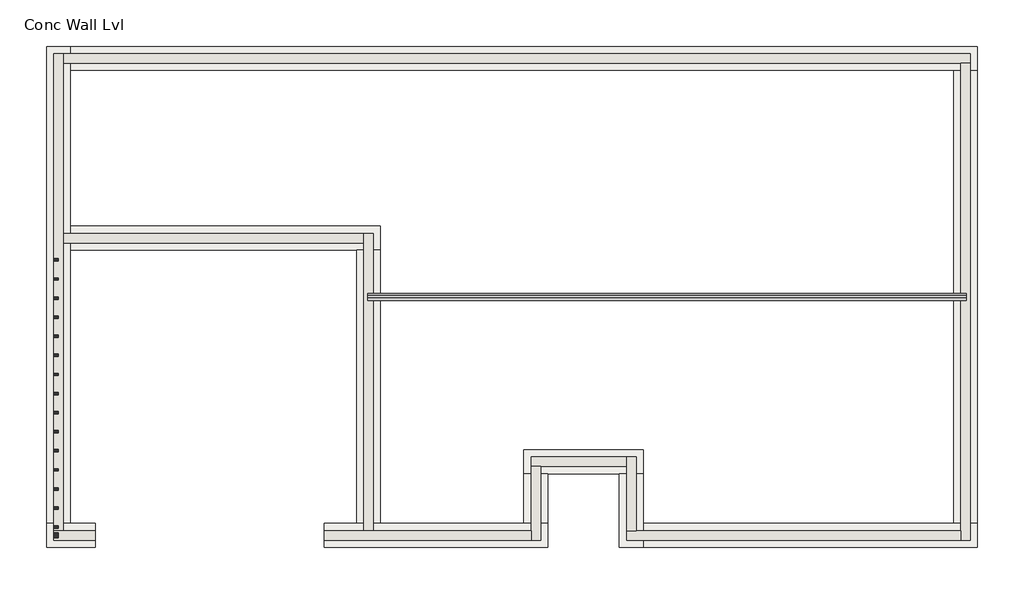
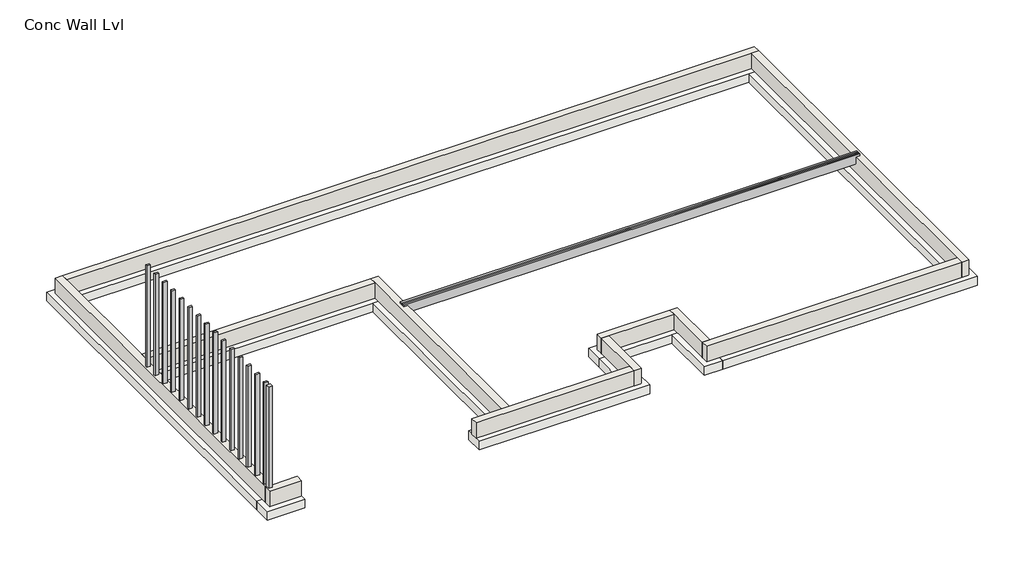
# One storey: 16 columns, 11 footings, 11 walls, 3 beams.
"""IFC4 building model written with IfcOpenShell, lengths in millimetres."""

import ifcopenshell
import ifcopenshell.guid

model = None  # the IFC model being written
_history = None  # IfcOwnerHistory: only IFC2X3 demands one
_inside = {}  # id of a spatial element -> (the spatial element, [elements in it])
_under = {}  # id of a project, library or spatial element -> (it, [spatial elements below it])
_declared = {}  # id of a project -> (the project, [libraries it declares])
_typed = {}  # id of a type object -> (the type object, [elements of that type])
_made_of = {}  # id of a material, layer set ... -> (it, [elements and type objects made of it])


def new_model(schema):
    """Start an empty IFC model of exactly this schema.

    Asked for "IFC4X3", IfcOpenShell would pick the latest addendum, in which some entities
    have other attributes; the version numbers below select the first issue.
    IFC2X3 requires an IfcOwnerHistory on every rooted entity: one is made here for all.
    """
    global model, _history
    if schema == "IFC4X3":
        model = ifcopenshell.file(schema_version=(4, 3, 0, 0))
    else:
        model = ifcopenshell.file(schema=schema)
    _inside.clear()
    _under.clear()
    _declared.clear()
    _typed.clear()
    _made_of.clear()
    _history = None
    if model.schema == "IFC2X3":
        org = make("IfcOrganization", Name="unknown")
        user = make(
            "IfcPersonAndOrganization",
            ThePerson=make("IfcPerson", FamilyName="unknown"),
            TheOrganization=org,
        )
        app = make(
            "IfcApplication",
            ApplicationDeveloper=org,
            Version="unknown",
            ApplicationFullName="unknown",
            ApplicationIdentifier="unknown",
        )
        _history = make(
            "IfcOwnerHistory",
            OwningUser=user,
            OwningApplication=app,
            ChangeAction="ADDED",
            CreationDate=0,
        )
    return model


def make(cls, **values):
    """One entity of the class cls with the attributes given. An attribute that is None is left unset."""
    return model.create_entity(
        cls, **{name: value for name, value in values.items() if value is not None}
    )


def rooted(cls, **values):
    """An entity with a GlobalId (a new one), such as an element, a storey or a relation."""
    return make(cls, GlobalId=ifcopenshell.guid.new(), OwnerHistory=_history, **values)


def si_unit(unit_type, name, prefix=None):
    """IfcSIUnit, for example si_unit("LENGTHUNIT", "METRE", prefix="MILLI")."""
    return make("IfcSIUnit", UnitType=unit_type, Prefix=prefix, Name=name)


def assignment(units):
    """IfcUnitAssignment: the units of a project."""
    return None if units is None else make("IfcUnitAssignment", Units=units)


def point(xyz):
    """IfcCartesianPoint."""
    return None if xyz is None else make("IfcCartesianPoint", Coordinates=xyz)


def direction(xyz):
    """IfcDirection."""
    return None if xyz is None else make("IfcDirection", DirectionRatios=xyz)


def frame(location, z_axis=None, x_axis=None):
    """IfcAxis2Placement3D, a coordinate frame: its origin and axes. An axis left out is left unset."""
    return make(
        "IfcAxis2Placement3D",
        Location=point(location),
        Axis=direction(z_axis),
        RefDirection=direction(x_axis),
    )


def origin():
    """The frame at (0, 0, 0) with its axes left unset."""
    return frame((0.0, 0.0, 0.0))


def place(relative_to, where):
    """IfcLocalPlacement: puts the frame where relative to a parent placement (None: the world)."""
    return make(
        "IfcLocalPlacement", PlacementRelTo=relative_to, RelativePlacement=where
    )


def context(
    kind, dimensions, precision=None, world=None, true_north=None, identifier=None
):
    """IfcGeometricRepresentationContext, for example the 3D "Model" context."""
    return make(
        "IfcGeometricRepresentationContext",
        ContextIdentifier=identifier,
        ContextType=kind,
        CoordinateSpaceDimension=dimensions,
        Precision=precision,
        WorldCoordinateSystem=world,
        TrueNorth=true_north,
    )


def project(units=None, contexts=None):
    """IfcProject with its units and contexts."""
    return rooted(
        "IfcProject",
        Name="project",
        RepresentationContexts=contexts,
        UnitsInContext=assignment(units),
    )


def spatial(cls, under=None, at=None, **own):
    """A site, building, storey or space (cls), placed at a placement, below another one or the project."""
    s = rooted(cls, ObjectPlacement=at, **own)
    if under is not None:
        _under.setdefault(under.id(), (under, []))[1].append(s)
    return s


def polyline(points):
    """IfcPolyline through the points."""
    return make("IfcPolyline", Points=[point(p) for p in points])


def outline(outer, holes=None, kind="AREA"):
    """IfcArbitraryClosedProfileDef: a profile drawn as a closed curve; with holes, ...WithVoids."""
    if holes is None:
        return make("IfcArbitraryClosedProfileDef", ProfileType=kind, OuterCurve=outer)
    return make(
        "IfcArbitraryProfileDefWithVoids",
        ProfileType=kind,
        OuterCurve=outer,
        InnerCurves=holes,
    )


def extrude(swept, where, along, depth):
    """IfcExtrudedAreaSolid: the profile swept, set in the frame where, extruded along a direction by depth."""
    return make(
        "IfcExtrudedAreaSolid",
        SweptArea=swept,
        Position=where,
        ExtrudedDirection=direction(along),
        Depth=depth,
    )


def faces_of(points, faces, orient=None, outer=None):
    """IfcFace entities. A face is a list of loops; a loop is a list of indices into points, from 0.

    orient and outer hold one flag for each loop. By default every Orientation is true, the
    first loop of a face is its IfcFaceOuterBound and the others are IfcFaceBound.
    """
    made = []
    for i, loops in enumerate(faces):
        bounds = []
        for j, loop in enumerate(loops):
            is_outer = j == 0 if outer is None else outer[i][j]
            bounds.append(
                make(
                    "IfcFaceOuterBound" if is_outer else "IfcFaceBound",
                    Bound=make("IfcPolyLoop", Polygon=[points[k] for k in loop]),
                    Orientation=True if orient is None else orient[i][j],
                )
            )
        made.append(make("IfcFace", Bounds=bounds))
    return made


def faceted_brep(points, faces, orient=None, outer=None, voids=None):
    """IfcFacetedBrep: a solid bounded by flat faces; with voids (closed shells), ...WithVoids."""
    shared = [point(p) for p in points]
    hull = make("IfcClosedShell", CfsFaces=faces_of(shared, faces, orient, outer))
    if voids is None:
        return make("IfcFacetedBrep", Outer=hull)
    return make(
        "IfcFacetedBrepWithVoids",
        Outer=hull,
        Voids=[
            make(cls, CfsFaces=faces_of(shared, fs, o, b)) for cls, fs, o, b in voids
        ],
    )


def shape(context_of_items, identifier, shape_type, items):
    """IfcShapeRepresentation: the items that make up one representation, for example the "Body"."""
    return make(
        "IfcShapeRepresentation",
        ContextOfItems=context_of_items,
        RepresentationIdentifier=identifier,
        RepresentationType=shape_type,
        Items=items,
    )


def source(mapping_origin, context_of_items, identifier, shape_type, items):
    """IfcRepresentationMap: a shape defined once, which mapped items show again and again."""
    return make(
        "IfcRepresentationMap",
        MappingOrigin=mapping_origin,
        MappedRepresentation=shape(context_of_items, identifier, shape_type, items),
    )


def transform(
    local_origin,
    x_axis=None,
    y_axis=None,
    z_axis=None,
    scale=None,
    scale2=None,
    scale3=None,
    uniform=True,
):
    """IfcCartesianTransformationOperator3D, or its non-uniform kind. x_axis, y_axis, z_axis: its Axis1, 2, 3."""
    if uniform:
        return make(
            "IfcCartesianTransformationOperator3D",
            Axis1=direction(x_axis),
            Axis2=direction(y_axis),
            LocalOrigin=point(local_origin),
            Scale=scale,
            Axis3=direction(z_axis),
        )
    return make(
        "IfcCartesianTransformationOperator3DnonUniform",
        Axis1=direction(x_axis),
        Axis2=direction(y_axis),
        LocalOrigin=point(local_origin),
        Scale=scale,
        Axis3=direction(z_axis),
        Scale2=scale2,
        Scale3=scale3,
    )


def mapped(mapping_source, mapping_target):
    """IfcMappedItem: shows the shape of a source again, moved by a transform."""
    return make(
        "IfcMappedItem", MappingSource=mapping_source, MappingTarget=mapping_target
    )


def made_of(thing, what):
    """Note that an element or type object is made of a material, layer set ...; save() writes the relation."""
    if what is not None:
        _made_of.setdefault(what.id(), (what, []))[1].append(thing)
    return thing


def element(
    cls,
    number,
    at=None,
    inside=None,
    cuts=None,
    type_object=None,
    material=None,
    context=None,
    identifier="Body",
    shape_type=None,
    held_by="IfcProductDefinitionShape",
    body=None,
    shapes=None,
    **own,
):
    """One element of the class cls, such as IfcWall. Its Tag is "e" and its number.

    at: its placement. inside: the storey or other place that contains it. cuts: it is an
    opening in that element (IfcRelVoidsElement). A single representation is given by context,
    identifier, shape_type and body (its items); several are given by shapes. held_by: the class
    of the entity that holds the representations. save() writes the other relations.
    """
    e = rooted(cls, Tag="e%d" % number, ObjectPlacement=at, **own)
    if body is not None:
        shapes = [shape(context, identifier, shape_type, body)]
    if shapes is not None:
        e.Representation = make(held_by, Representations=shapes)
    if inside is not None:
        _inside.setdefault(inside.id(), (inside, []))[1].append(e)
    if cuts is not None:
        rooted(
            "IfcRelVoidsElement", RelatingBuildingElement=cuts, RelatedOpeningElement=e
        )
    if type_object is not None:
        _typed.setdefault(type_object.id(), (type_object, []))[1].append(e)
    return made_of(e, material)


def aggregate(whole, parts):
    """IfcRelAggregates: a whole, such as a stair, and the parts it consists of."""
    return rooted("IfcRelAggregates", RelatingObject=whole, RelatedObjects=parts)


def save(model, path):
    """Write the relations noted so far, then the file.

    IfcRelAggregates (storeys below a building ...), IfcRelContainedInSpatialStructure (elements
    in a storey), IfcRelDefinesByType, IfcRelAssociatesMaterial and IfcRelDeclares: one each for
    every whole, place, type object, material and project.
    """
    for whole, parts in _under.values():
        aggregate(whole, parts)
    for where, things in _inside.values():
        rooted(
            "IfcRelContainedInSpatialStructure",
            RelatedElements=things,
            RelatingStructure=where,
        )
    for kind, things in _typed.values():
        rooted("IfcRelDefinesByType", RelatedObjects=things, RelatingType=kind)
    for what, things in _made_of.values():
        rooted("IfcRelAssociatesMaterial", RelatedObjects=things, RelatingMaterial=what)
    for by, libraries in _declared.values():
        rooted("IfcRelDeclares", RelatingContext=by, RelatedDefinitions=libraries)
    model.write(path)


def beam_bcf194da(model_context):
    return source(origin(), model_context, "Body", "SweptSolid", [
        extrude(outline(polyline([(6302.375, 25.4), (6302.375, -25.4), (-6429.375, -25.4), (-6429.375, 25.4), (6302.375, 25.4)])), frame((0.0, 0.0, -127.0), z_axis=(0.0, 0.0, 1.0), x_axis=(1.0, 0.0, 0.0)), (0.0, 0.0, 1.0), 254.0),
    ])


def timber_column_4ee0a357(model_context):
    return source(origin(), model_context, "Body", "SweptSolid", [
        extrude(outline(polyline([(25.4, 50.8), (25.4, -50.8), (-25.4, -50.8), (-25.4, 50.8), (25.4, 50.8)])), frame((0.0, 0.0, -319.88125), z_axis=(0.0, 0.0, 1.0), x_axis=(1.0, 0.0, 0.0)), (0.0, 0.0, 1.0), 2986.88125),
    ])


def timber_column_8a3ad47c(model_context):
    return source(origin(), model_context, "Body", "SweptSolid", [
        extrude(outline(polyline([(50.8, 50.8), (50.8, -50.8), (-50.8, -50.8), (-50.8, 50.8), (50.8, 50.8)])), frame((0.0, 0.0, -319.88125), z_axis=(0.0, 0.0, 1.0), x_axis=(1.0, 0.0, 0.0)), (0.0, 0.0, 1.0), 2986.88125),
    ])


model = new_model("IFC4")

# Units and contexts
model_context = context("Model", 3, world=origin())
ifc_project = project(units=[si_unit("LENGTHUNIT", "METRE", prefix="MILLI")], contexts=[model_context])

# Site, building, storey
site = spatial("IfcSite", under=ifc_project)
building = spatial("IfcBuilding", under=site)
storey = spatial("IfcBuildingStorey", under=building, Name="Conc Wall Lvl", Elevation=-370.68125)

# Beams
placement = place(None, origin())
beam_shape = beam_bcf194da(model_context)
element("IfcBeam", 1, ObjectType="Dimension Lumber : BLDG 6241 2x10\" Beam", at=placement, inside=storey, context=model_context, shape_type="MappedRepresentation", body=[
    mapped(beam_shape, transform((-4812.289829, 26.1284114, -446.88125), x_axis=(-1.0, 0.0, 0.0), y_axis=(0.0, -1.0, 0.0), z_axis=(0.0, 0.0, 1.0))),
])
element("IfcBeam", 2, ObjectType="Dimension Lumber : BLDG 6241 2x10\" Beam", at=placement, inside=storey, context=model_context, shape_type="MappedRepresentation", body=[
    mapped(beam_shape, transform((-4812.289829, 76.9284114, -446.88125), x_axis=(-1.0, 0.0, 0.0), y_axis=(0.0, -1.0, 0.0), z_axis=(0.0, 0.0, 1.0))),
])
element("IfcBeam", 3, ObjectType="Dimension Lumber : BLDG 6241 2x10\" Beam", at=placement, inside=storey, context=model_context, shape_type="MappedRepresentation", body=[
    mapped(beam_shape, transform((-4812.289829, -24.6715886, -446.88125), x_axis=(-1.0, 0.0, 0.0), y_axis=(0.0, -1.0, 0.0), z_axis=(0.0, 0.0, 1.0))),
])

# Columns
timber_column_shape = timber_column_4ee0a357(model_context)
element("IfcColumn", 4, ObjectType="Timber-Column : BLDG 6241 Wall Struds 2\"x4\"", at=placement, inside=storey, context=model_context, shape_type="MappedRepresentation", body=[
    mapped(timber_column_shape, transform((-17750.414829, 813.5284114, 0.0), x_axis=(0.0, 1.0, 0.0), y_axis=(-1.0, 0.0, 0.0), z_axis=(0.0, 0.0, 1.0))),
])
element("IfcColumn", 5, ObjectType="Timber-Column : BLDG 6241 Wall Struds 2\"x4\"", at=placement, inside=storey, context=model_context, shape_type="MappedRepresentation", body=[
    mapped(timber_column_shape, transform((-17750.414829, 407.1284114, 0.0), x_axis=(0.0, 1.0, 0.0), y_axis=(-1.0, 0.0, 0.0), z_axis=(0.0, 0.0, 1.0))),
])
element("IfcColumn", 6, ObjectType="Timber-Column : BLDG 6241 Wall Struds 2\"x4\"", at=placement, inside=storey, context=model_context, shape_type="MappedRepresentation", body=[
    mapped(timber_column_shape, transform((-17750.414829, 0.7284114, 0.0), x_axis=(0.0, 1.0, 0.0), y_axis=(-1.0, 0.0, 0.0), z_axis=(0.0, 0.0, 1.0))),
])
element("IfcColumn", 7, ObjectType="Timber-Column : BLDG 6241 Wall Struds 2\"x4\"", at=placement, inside=storey, context=model_context, shape_type="MappedRepresentation", body=[
    mapped(timber_column_shape, transform((-17750.414829, -405.6715886, 0.0), x_axis=(0.0, 1.0, 0.0), y_axis=(-1.0, 0.0, 0.0), z_axis=(0.0, 0.0, 1.0))),
])
element("IfcColumn", 8, ObjectType="Timber-Column : BLDG 6241 Wall Struds 2\"x4\"", at=placement, inside=storey, context=model_context, shape_type="MappedRepresentation", body=[
    mapped(timber_column_shape, transform((-17750.414829, -812.0715886, 0.0), x_axis=(0.0, 1.0, 0.0), y_axis=(-1.0, 0.0, 0.0), z_axis=(0.0, 0.0, 1.0))),
])
element("IfcColumn", 9, ObjectType="Timber-Column : BLDG 6241 Wall Struds 2\"x4\"", at=placement, inside=storey, context=model_context, shape_type="MappedRepresentation", body=[
    mapped(timber_column_shape, transform((-17750.414829, -1218.4715886, 0.0), x_axis=(0.0, 1.0, 0.0), y_axis=(-1.0, 0.0, 0.0), z_axis=(0.0, 0.0, 1.0))),
])
element("IfcColumn", 10, ObjectType="Timber-Column : BLDG 6241 Wall Struds 2\"x4\"", at=placement, inside=storey, context=model_context, shape_type="MappedRepresentation", body=[
    mapped(timber_column_shape, transform((-17750.414829, -1624.8715886, 0.0), x_axis=(0.0, 1.0, 0.0), y_axis=(-1.0, 0.0, 0.0), z_axis=(0.0, 0.0, 1.0))),
])
element("IfcColumn", 11, ObjectType="Timber-Column : BLDG 6241 Wall Struds 2\"x4\"", at=placement, inside=storey, context=model_context, shape_type="MappedRepresentation", body=[
    mapped(timber_column_shape, transform((-17750.414829, -2031.2715886, 0.0), x_axis=(0.0, 1.0, 0.0), y_axis=(-1.0, 0.0, 0.0), z_axis=(0.0, 0.0, 1.0))),
])
element("IfcColumn", 12, ObjectType="Timber-Column : BLDG 6241 Wall Struds 2\"x4\"", at=placement, inside=storey, context=model_context, shape_type="MappedRepresentation", body=[
    mapped(timber_column_shape, transform((-17750.414829, -2437.6715886, 0.0), x_axis=(0.0, 1.0, 0.0), y_axis=(-1.0, 0.0, 0.0), z_axis=(0.0, 0.0, 1.0))),
])
element("IfcColumn", 13, ObjectType="Timber-Column : BLDG 6241 Wall Struds 2\"x4\"", at=placement, inside=storey, context=model_context, shape_type="MappedRepresentation", body=[
    mapped(timber_column_shape, transform((-17750.414829, -2844.0715886, 0.0), x_axis=(0.0, 1.0, 0.0), y_axis=(-1.0, 0.0, 0.0), z_axis=(0.0, 0.0, 1.0))),
])
element("IfcColumn", 14, ObjectType="Timber-Column : BLDG 6241 Wall Struds 2\"x4\"", at=placement, inside=storey, context=model_context, shape_type="MappedRepresentation", body=[
    mapped(timber_column_shape, transform((-17750.414829, -3250.4715886, 0.0), x_axis=(0.0, 1.0, 0.0), y_axis=(-1.0, 0.0, 0.0), z_axis=(0.0, 0.0, 1.0))),
])
element("IfcColumn", 15, ObjectType="Timber-Column : BLDG 6241 Wall Struds 2\"x4\"", at=placement, inside=storey, context=model_context, shape_type="MappedRepresentation", body=[
    mapped(timber_column_shape, transform((-17750.414829, -3656.8715886, 0.0), x_axis=(0.0, 1.0, 0.0), y_axis=(-1.0, 0.0, 0.0), z_axis=(0.0, 0.0, 1.0))),
])
element("IfcColumn", 16, ObjectType="Timber-Column : BLDG 6241 Wall Struds 2\"x4\"", at=placement, inside=storey, context=model_context, shape_type="MappedRepresentation", body=[
    mapped(timber_column_shape, transform((-17750.414829, -4063.2715886, 0.0), x_axis=(0.0, 1.0, 0.0), y_axis=(-1.0, 0.0, 0.0), z_axis=(0.0, 0.0, 1.0))),
])
element("IfcColumn", 17, ObjectType="Timber-Column : BLDG 6241 Wall Struds 2\"x4\"", at=placement, inside=storey, context=model_context, shape_type="MappedRepresentation", body=[
    mapped(timber_column_shape, transform((-17750.414829, -4469.6715886, 0.0), x_axis=(0.0, 1.0, 0.0), y_axis=(-1.0, 0.0, 0.0), z_axis=(0.0, 0.0, 1.0))),
])
element("IfcColumn", 18, ObjectType="Timber-Column : BLDG 6241 Wall Struds 2\"x4\"", at=placement, inside=storey, context=model_context, shape_type="MappedRepresentation", body=[
    mapped(timber_column_shape, transform((-17750.414829, -4876.0715886, 0.0), x_axis=(0.0, 1.0, 0.0), y_axis=(-1.0, 0.0, 0.0), z_axis=(0.0, 0.0, 1.0))),
])
timber_column_2_shape = timber_column_8a3ad47c(model_context)
element("IfcColumn", 19, ObjectType="Timber-Column : BLDG 6241 Wall Struds 4\"x4\"", at=placement, inside=storey, context=model_context, shape_type="MappedRepresentation", body=[
    mapped(timber_column_2_shape, transform((-17750.414829, -5053.8715886, 0.0), x_axis=(1.0, 0.0, 0.0), y_axis=(0.0, 1.0, 0.0), z_axis=(0.0, 0.0, 1.0))),
])

# Footings
element("IfcFooting", 20, ObjectType="BLDG Conc Footing - 20\" x 10\"", at=placement, inside=storey, context=model_context, shape_type="Brep", body=[
    faceted_brep([(-16915.389829, -4799.8715886, -827.88125), (-16915.389829, -5307.8715886, -827.88125), (-16915.389829, -5307.8715886, -1081.88125), (-16915.389829, -4799.8715886, -1081.88125), (-17445.614829, -4799.8715886, -827.88125), (-17953.614829, -4799.8715886, -827.88125), (-17953.614829, -5307.8715886, -827.88125), (-17953.614829, -5307.8715886, -1081.88125), (-17953.614829, -4799.8715886, -1081.88125), (-17445.614829, -4799.8715886, -1081.88125)], [[[0, 1, 2, 3]], [[0, 4, 5, 6, 1]], [[2, 1, 6, 7]], [[3, 2, 7, 8, 9]], [[0, 3, 9, 8, 5, 4]], [[6, 5, 8, 7]]]),
])
element("IfcFooting", 21, ObjectType="BLDG Conc Footing - 20\" x 10\"", at=placement, inside=storey, context=model_context, shape_type="Brep", body=[
    faceted_brep([(-17445.614829, 5360.1284114, -827.88125), (-17953.614829, 5360.1284114, -827.88125), (-17953.614829, -4799.8715886, -827.88125), (-17445.614829, -4799.8715886, -827.88125), (-17445.614829, 1023.0784114, -827.88125), (-17445.614829, 1531.0784114, -827.88125), (-17445.614829, 4852.1284114, -827.88125), (-17953.614829, 5360.1284114, -1081.88125), (-17953.614829, -4799.8715886, -1081.88125), (-17445.614829, 5360.1284114, -1081.88125), (-17445.614829, 4852.1284114, -1081.88125), (-17445.614829, 1531.0784114, -1081.88125), (-17445.614829, 1023.0784114, -1081.88125), (-17445.614829, -4799.8715886, -1081.88125)], [[[0, 1, 2, 3, 4, 5, 6]], [[1, 7, 8, 2]], [[7, 9, 10, 11, 12, 13, 8]], [[9, 0, 6, 5, 4, 3, 13, 12, 11, 10]], [[3, 2, 8, 13]], [[1, 0, 9, 7]]]),
])
element("IfcFooting", 22, ObjectType="BLDG Conc Footing - 20\" x 10\"", at=placement, inside=storey, context=model_context, shape_type="Brep", body=[
    faceted_brep([(-10847.964829, 1531.0784114, -827.88125), (-17445.614829, 1531.0784114, -827.88125), (-17445.614829, 1023.0784114, -827.88125), (-11355.964829, 1023.0784114, -827.88125), (-10847.964829, 1023.0784114, -827.88125), (-10847.964829, 1023.0784114, -1081.88125), (-17445.614829, 1023.0784114, -1081.88125), (-11355.964829, 1023.0784114, -1081.88125), (-10847.964829, 1531.0784114, -1081.88125), (-17445.614829, 1531.0784114, -1081.88125)], [[[0, 1, 2, 3, 4]], [[5, 4, 3, 2, 6, 7]], [[8, 5, 7, 6, 9]], [[0, 8, 9, 1]], [[2, 1, 9, 6]], [[0, 4, 5, 8]]]),
])
element("IfcFooting", 23, ObjectType="BLDG Conc Footing - 20\" x 10\"", at=placement, inside=storey, context=model_context, shape_type="SweptSolid", body=[
    extrude(outline(polyline([(-10847.964829, -4799.8715886), (-11355.964829, -4799.8715886), (-11355.964829, 1023.0784114), (-10847.964829, 1023.0784114), (-10847.964829, -4799.8715886)])), frame((0.0, 0.0, -1081.88125), z_axis=(0.0, 0.0, 1.0), x_axis=(1.0, 0.0, 0.0)), (0.0, 0.0, 1.0), 254.0),
])
element("IfcFooting", 24, ObjectType="BLDG Conc Footing - 20\" x 10\"", at=placement, inside=storey, context=model_context, shape_type="Brep", body=[
    faceted_brep([(-12038.589829, -5307.8715886, -827.88125), (-12038.589829, -4799.8715886, -827.88125), (-12038.589829, -4799.8715886, -1081.88125), (-12038.589829, -5307.8715886, -1081.88125), (-7285.614829, -4799.8715886, -827.88125), (-7793.614829, -4799.8715886, -827.88125), (-10847.964829, -4799.8715886, -827.88125), (-11355.964829, -4799.8715886, -827.88125), (-7285.614829, -5307.8715886, -827.88125), (-7285.614829, -5307.8715886, -1081.88125), (-7285.614829, -4799.8715886, -1081.88125), (-11355.964829, -4799.8715886, -1081.88125), (-10847.964829, -4799.8715886, -1081.88125), (-7793.614829, -4799.8715886, -1081.88125)], [[[0, 1, 2, 3]], [[4, 5, 6, 7, 1, 0, 8]], [[9, 8, 0, 3]], [[10, 9, 3, 2, 11, 12, 13]], [[4, 10, 13, 12, 11, 2, 1, 7, 6, 5]], [[4, 8, 9, 10]]]),
])
element("IfcFooting", 25, ObjectType="BLDG Conc Footing - 20\" x 10\"", at=placement, inside=storey, context=model_context, shape_type="Brep", body=[
    faceted_brep([(-5253.614829, -3231.4215886, -827.88125), (-7793.614829, -3231.4215886, -827.88125), (-7793.614829, -3739.4215886, -827.88125), (-7285.614829, -3739.4215886, -827.88125), (-5761.614829, -3739.4215886, -827.88125), (-5253.614829, -3739.4215886, -827.88125), (-5253.614829, -3739.4215886, -1081.88125), (-7793.614829, -3739.4215886, -1081.88125), (-7285.614829, -3739.4215886, -1081.88125), (-5761.614829, -3739.4215886, -1081.88125), (-5253.614829, -3231.4215886, -1081.88125), (-7793.614829, -3231.4215886, -1081.88125)], [[[0, 1, 2, 3, 4, 5]], [[6, 5, 4, 3, 2, 7, 8, 9]], [[10, 6, 9, 8, 7, 11]], [[0, 10, 11, 1]], [[0, 5, 6, 10]], [[2, 1, 11, 7]]]),
])
element("IfcFooting", 26, ObjectType="BLDG Conc Footing - 20\" x 10\"", at=placement, inside=storey, context=model_context, shape_type="Brep", body=[
    faceted_brep([(-5761.614829, -5307.8715886, -827.88125), (-5253.614829, -5307.8715886, -827.88125), (-5253.614829, -4799.8715886, -827.88125), (-5253.614829, -3739.4215886, -827.88125), (-5761.614829, -3739.4215886, -827.88125), (-5761.614829, -5307.8715886, -1081.88125), (-5761.614829, -3739.4215886, -1081.88125), (-5253.614829, -5307.8715886, -1081.88125), (-5253.614829, -3739.4215886, -1081.88125), (-5253.614829, -4799.8715886, -1081.88125)], [[[0, 1, 2, 3, 4]], [[5, 0, 4, 6]], [[7, 5, 6, 8, 9]], [[1, 7, 9, 8, 3, 2]], [[4, 3, 8, 6]], [[1, 0, 5, 7]]]),
])
element("IfcFooting", 27, ObjectType="BLDG Conc Footing - 20\" x 10\"", at=placement, inside=storey, context=model_context, shape_type="Brep", body=[
    faceted_brep([(1858.385171, -5307.8715886, -827.88125), (1858.385171, -4799.8715886, -827.88125), (1350.385171, -4799.8715886, -827.88125), (-5253.614829, -4799.8715886, -827.88125), (-5253.614829, -5307.8715886, -827.88125), (1858.385171, -5307.8715886, -1081.88125), (-5253.614829, -5307.8715886, -1081.88125), (1858.385171, -4799.8715886, -1081.88125), (-5253.614829, -4799.8715886, -1081.88125), (1350.385171, -4799.8715886, -1081.88125)], [[[0, 1, 2, 3, 4]], [[5, 0, 4, 6]], [[7, 5, 6, 8, 9]], [[1, 7, 9, 8, 3, 2]], [[4, 3, 8, 6]], [[1, 0, 5, 7]]]),
])
element("IfcFooting", 28, ObjectType="BLDG Conc Footing - 20\" x 10\"", at=placement, inside=storey, context=model_context, shape_type="SweptSolid", body=[
    extrude(outline(polyline([(-7285.614829, -4799.8715886), (-7793.614829, -4799.8715886), (-7793.614829, -3739.4215886), (-7285.614829, -3739.4215886), (-7285.614829, -4799.8715886)])), frame((0.0, 0.0, -1081.88125), z_axis=(0.0, 0.0, 1.0), x_axis=(1.0, 0.0, 0.0)), (0.0, 0.0, 1.0), 254.0),
])
element("IfcFooting", 29, ObjectType="BLDG Conc Footing - 20\" x 10\"", at=placement, inside=storey, context=model_context, shape_type="Brep", body=[
    faceted_brep([(1858.385171, 4852.1284114, -827.88125), (1858.385171, 5360.1284114, -827.88125), (-17445.614829, 5360.1284114, -827.88125), (-17445.614829, 4852.1284114, -827.88125), (1350.385171, 4852.1284114, -827.88125), (1858.385171, 5360.1284114, -1081.88125), (-17445.614829, 5360.1284114, -1081.88125), (1858.385171, 4852.1284114, -1081.88125), (1350.385171, 4852.1284114, -1081.88125), (-17445.614829, 4852.1284114, -1081.88125)], [[[0, 1, 2, 3, 4]], [[1, 5, 6, 2]], [[5, 7, 8, 9, 6]], [[7, 0, 4, 3, 9, 8]], [[3, 2, 6, 9]], [[1, 0, 7, 5]]]),
])
element("IfcFooting", 30, ObjectType="BLDG Conc Footing - 20\" x 10\"", at=placement, inside=storey, context=model_context, shape_type="SweptSolid", body=[
    extrude(outline(polyline([(1858.385171, -4799.8715886), (1350.385171, -4799.8715886), (1350.385171, 4852.1284114), (1858.385171, 4852.1284114), (1858.385171, -4799.8715886)])), frame((0.0, 0.0, -1081.88125), z_axis=(0.0, 0.0, 1.0), x_axis=(1.0, 0.0, 0.0)), (0.0, 0.0, 1.0), 254.0),
])

# Walls
element("IfcWall", 31, ObjectType="BLDG 6241 Conc Wall - 8\"", at=placement, inside=storey, context=model_context, shape_type="Brep", body=[
    faceted_brep([(-16915.389829, -4952.2715886, -827.88125), (-17598.014829, -4952.2715886, -827.88125), (-17801.214829, -4952.2715886, -827.88125), (-17801.214829, -4952.2715886, -370.68125), (-17598.014829, -4952.2715886, -370.68125), (-16915.389829, -4952.2715886, -370.68125), (-16915.389829, -5155.4715886, -827.88125), (-16915.389829, -5155.4715886, -370.68125), (-17801.214829, -5155.4715886, -370.68125), (-17801.214829, -5155.4715886, -827.88125)], [[[0, 1, 2, 3, 4, 5]], [[6, 7, 8, 9]], [[2, 1, 0, 6, 9]], [[5, 4, 3, 8, 7]], [[0, 5, 7, 6]], [[3, 2, 9, 8]]]),
])
element("IfcWall", 32, ObjectType="BLDG 6241 Conc Wall - 8\"", at=placement, inside=storey, context=model_context, shape_type="Brep", body=[
    faceted_brep([(-17598.014829, -4952.2715886, -827.88125), (-17598.014829, 1175.4784114, -827.88125), (-17598.014829, 1378.6784114, -827.88125), (-17598.014829, 5004.5284114, -827.88125), (-17598.014829, 5207.7284114, -827.88125), (-17598.014829, 5207.7284114, -370.68125), (-17598.014829, 5004.5284114, -370.68125), (-17598.014829, 1378.6784114, -370.68125), (-17598.014829, 1175.4784114, -370.68125), (-17598.014829, -4952.2715886, -370.68125), (-17801.214829, -4952.2715886, -827.88125), (-17801.214829, -4952.2715886, -370.68125), (-17801.214829, 5207.7284114, -370.68125), (-17801.214829, 5207.7284114, -827.88125)], [[[0, 1, 2, 3, 4, 5, 6, 7, 8, 9]], [[10, 11, 12, 13]], [[4, 3, 2, 1, 0, 10, 13]], [[9, 8, 7, 6, 5, 12, 11]], [[0, 9, 11, 10]], [[5, 4, 13, 12]]]),
])
element("IfcWall", 33, ObjectType="BLDG 6241 Conc Wall - 8\"", at=placement, inside=storey, context=model_context, shape_type="Brep", body=[
    faceted_brep([(-17598.014829, 5004.5284114, -827.88125), (1502.785171, 5004.5284114, -827.88125), (1705.985171, 5004.5284114, -827.88125), (1705.985171, 5004.5284114, -370.68125), (1502.785171, 5004.5284114, -370.68125), (-17598.014829, 5004.5284114, -370.68125), (-17598.014829, 5207.7284114, -827.88125), (-17598.014829, 5207.7284114, -370.68125), (1705.985171, 5207.7284114, -370.68125), (1705.985171, 5207.7284114, -827.88125)], [[[0, 1, 2, 3, 4, 5]], [[6, 7, 8, 9]], [[2, 1, 0, 6, 9]], [[5, 4, 3, 8, 7]], [[0, 5, 7, 6]], [[3, 2, 9, 8]]]),
])
element("IfcWall", 34, ObjectType="BLDG 6241 Conc Wall - 8\"", at=placement, inside=storey, context=model_context, shape_type="Brep", body=[
    faceted_brep([(1502.785171, 5004.5284114, -827.88125), (1502.785171, -4952.2715886, -827.88125), (1502.785171, -5155.4715886, -827.88125), (1502.785171, -5155.4715886, -370.68125), (1502.785171, -4952.2715886, -370.68125), (1502.785171, 5004.5284114, -370.68125), (1705.985171, 5004.5284114, -827.88125), (1705.985171, 5004.5284114, -370.68125), (1705.985171, -5155.4715886, -370.68125), (1705.985171, -5155.4715886, -827.88125)], [[[0, 1, 2, 3, 4, 5]], [[6, 7, 8, 9]], [[2, 1, 0, 6, 9]], [[5, 4, 3, 8, 7]], [[0, 5, 7, 6]], [[3, 2, 9, 8]]]),
])
element("IfcWall", 35, ObjectType="BLDG 6241 Conc Wall - 8\"", at=placement, inside=storey, context=model_context, shape_type="Brep", body=[
    faceted_brep([(1502.785171, -4952.2715886, -827.88125), (-5406.014829, -4952.2715886, -827.88125), (-5609.214829, -4952.2715886, -827.88125), (-5609.214829, -4952.2715886, -370.68125), (-5406.014829, -4952.2715886, -370.68125), (1502.785171, -4952.2715886, -370.68125), (1502.785171, -5155.4715886, -827.88125), (1502.785171, -5155.4715886, -370.68125), (-5609.214829, -5155.4715886, -370.68125), (-5609.214829, -5155.4715886, -827.88125)], [[[0, 1, 2, 3, 4, 5]], [[6, 7, 8, 9]], [[2, 1, 0, 6, 9]], [[5, 4, 3, 8, 7]], [[0, 5, 7, 6]], [[3, 2, 9, 8]]]),
])
element("IfcWall", 36, ObjectType="BLDG 6241 Conc Wall - 8\"", at=placement, inside=storey, context=model_context, shape_type="Brep", body=[
    faceted_brep([(-5406.014829, -4952.2715886, -827.88125), (-5406.014829, -3383.8215886, -827.88125), (-5406.014829, -3383.8215886, -370.68125), (-5406.014829, -4952.2715886, -370.68125), (-5609.214829, -4952.2715886, -827.88125), (-5609.214829, -4952.2715886, -370.68125), (-5609.214829, -3587.0215886, -370.68125), (-5609.214829, -3383.8215886, -370.68125), (-5609.214829, -3383.8215886, -827.88125), (-5609.214829, -3587.0215886, -827.88125)], [[[0, 1, 2, 3]], [[4, 5, 6, 7, 8, 9]], [[1, 0, 4, 9, 8]], [[3, 2, 7, 6, 5]], [[0, 3, 5, 4]], [[2, 1, 8, 7]]]),
])
element("IfcWall", 37, ObjectType="BLDG 6241 Conc Wall - 8\"", at=placement, inside=storey, context=model_context, shape_type="Brep", body=[
    faceted_brep([(-5609.214829, -3383.8215886, -827.88125), (-7641.214829, -3383.8215886, -827.88125), (-7641.214829, -3383.8215886, -370.68125), (-5609.214829, -3383.8215886, -370.68125), (-5609.214829, -3587.0215886, -827.88125), (-5609.214829, -3587.0215886, -370.68125), (-7438.014829, -3587.0215886, -370.68125), (-7641.214829, -3587.0215886, -370.68125), (-7641.214829, -3587.0215886, -827.88125), (-7438.014829, -3587.0215886, -827.88125)], [[[0, 1, 2, 3]], [[4, 5, 6, 7, 8, 9]], [[1, 0, 4, 9, 8]], [[3, 2, 7, 6, 5]], [[0, 3, 5, 4]], [[2, 1, 8, 7]]]),
])
element("IfcWall", 38, ObjectType="BLDG 6241 Conc Wall - 8\"", at=placement, inside=storey, context=model_context, shape_type="Brep", body=[
    faceted_brep([(-7641.214829, -3587.0215886, -827.88125), (-7641.214829, -4952.2715886, -827.88125), (-7641.214829, -5155.4715886, -827.88125), (-7641.214829, -5155.4715886, -370.68125), (-7641.214829, -4952.2715886, -370.68125), (-7641.214829, -3587.0215886, -370.68125), (-7438.014829, -3587.0215886, -827.88125), (-7438.014829, -3587.0215886, -370.68125), (-7438.014829, -5155.4715886, -370.68125), (-7438.014829, -5155.4715886, -827.88125)], [[[0, 1, 2, 3, 4, 5]], [[6, 7, 8, 9]], [[2, 1, 0, 6, 9]], [[5, 4, 3, 8, 7]], [[0, 5, 7, 6]], [[3, 2, 9, 8]]]),
])
element("IfcWall", 39, ObjectType="BLDG 6241 Conc Wall - 8\"", at=placement, inside=storey, context=model_context, shape_type="Brep", body=[
    faceted_brep([(-7641.214829, -4952.2715886, -827.88125), (-11000.364829, -4952.2715886, -827.88125), (-11203.564829, -4952.2715886, -827.88125), (-12038.589829, -4952.2715886, -827.88125), (-12038.589829, -4952.2715886, -370.68125), (-11203.564829, -4952.2715886, -370.68125), (-11000.364829, -4952.2715886, -370.68125), (-7641.214829, -4952.2715886, -370.68125), (-7641.214829, -5155.4715886, -827.88125), (-7641.214829, -5155.4715886, -370.68125), (-12038.589829, -5155.4715886, -370.68125), (-12038.589829, -5155.4715886, -827.88125)], [[[0, 1, 2, 3, 4, 5, 6, 7]], [[8, 9, 10, 11]], [[3, 2, 1, 0, 8, 11]], [[4, 3, 11, 10]], [[7, 6, 5, 4, 10, 9]], [[0, 7, 9, 8]]]),
])
element("IfcWall", 40, ObjectType="BLDG 6241 Conc Wall - 8\"", at=placement, inside=storey, context=model_context, shape_type="Brep", body=[
    faceted_brep([(-11000.364829, -4952.2715886, -827.88125), (-11000.364829, 1378.6784114, -827.88125), (-11000.364829, 1378.6784114, -370.68125), (-11000.364829, -4952.2715886, -370.68125), (-11203.564829, -4952.2715886, -827.88125), (-11203.564829, -4952.2715886, -370.68125), (-11203.564829, 1175.4784114, -370.68125), (-11203.564829, 1378.6784114, -370.68125), (-11203.564829, 1378.6784114, -827.88125), (-11203.564829, 1175.4784114, -827.88125)], [[[0, 1, 2, 3]], [[4, 5, 6, 7, 8, 9]], [[1, 0, 4, 9, 8]], [[3, 2, 7, 6, 5]], [[0, 3, 5, 4]], [[2, 1, 8, 7]]]),
])
element("IfcWall", 41, ObjectType="BLDG 6241 Conc Wall - 8\"", at=placement, inside=storey, context=model_context, shape_type="SweptSolid", body=[
    extrude(outline(polyline([(-17598.014829, 1378.6784114), (-11203.564829, 1378.6784114), (-11203.564829, 1175.4784114), (-17598.014829, 1175.4784114), (-17598.014829, 1378.6784114)])), frame((0.0, 0.0, -827.88125), z_axis=(0.0, 0.0, 1.0), x_axis=(1.0, 0.0, 0.0)), (0.0, 0.0, 1.0), 457.2),
])

save(model, "model.ifc")

# Revit data of these elements
# Project information
#   Project Issue Date = "Issue Date"
#   Project Status = "Project Status"
#   Client Name = "Owner"
#   Project Address = "Enter address here"
#   Project Name = "Project Name"
#   Project Number = "Project Number"
# Grids (mm)
#   "X": line (-20839.361, 26.128) -> (5817.21, 26.128)
#   "1": line (-17801.215, 8272.214) -> (-17801.215, -7229.778)
#   "2": line (-11152.765, 8272.214) -> (-11152.765, -7229.778)
#   "3": line (-7438.015, 8272.214) -> (-7438.015, -7229.778)
#   "4": line (-6828.415, 8272.214) -> (-6828.415, -7229.778)
#   "5": line (-5609.215, 8272.214) -> (-5609.215, -7229.778)
#   "6": line (-2561.215, 8272.214) -> (-2561.215, -7229.778)
#   "7": line (-1951.615, 8272.214) -> (-1951.615, -7229.778)
#   "8": line (1705.985, 8272.214) -> (1705.985, -7229.778)
#   "A": line (-20839.361, 5207.728) -> (5817.21, 5207.728)
#   "B": line (-20839.361, 1226.278) -> (5817.21, 1226.278)
#   "C": line (-20839.361, -837.472) -> (5817.21, -837.472)
#   "D": line (-20839.361, -3529.872) -> (5817.21, -3529.872)
#   "E": line (-20839.361, -5053.872) -> (5817.21, -5053.872)
#   "G": line (-20839.361, -5155.472) -> (5817.21, -5155.472)
# Type "Dimension Lumber : BLDG 6241 2x10\" Beam"
#   Assembly Code = "B10"
#   A = 0.273472 SF
#   Length [instance default] = 5' - 0"
#   b = 0' - 2"
#   d = 0' - 10"
#   Structural Material [instance default] = Softwood, Lumber
# Type "Timber-Column : BLDG 6241 Wall Struds 2\"x4\""
#   Assembly Code = "B10"
#   A = 0.140625 SF
#   b = 0' - 2"
#   d = 0' - 4"
#   Structural Material [instance default] = Softwood, Lumber
# Type "Timber-Column : BLDG 6241 Wall Struds 4\"x4\""
#   Assembly Code = "B10"
#   A = 0.140625 SF
#   b = 0' - 4"
#   d = 0' - 4"
#   Structural Material [instance default] = Softwood, Lumber
# Type "BLDG Conc Footing - 20\" x 10\""
#   Assembly Code = "A1010110"
# Type "BLDG 6241 Conc Wall - 8\""
#   Assembly Code = "B2010"
#   Layers, outside or top first: 0' - 8" "BLDG 6241 Concrete(3500 psi)" (function 1)
# Elements 1, 2, 3 (IfcBeam, "Dimension Lumber : BLDG 6241 2x10\" Beam")
#   Comments = ""
#   Structural Material = Softwood, Lumber
#   Phase Created = New Construction
#   Materials on its faces: "Softwood, Lumber"
# Elements 4, 5, 6, 7, 8, 9, 10, 11, 12, 13, 14, 15, 16, 17, 18 (IfcColumn, "Timber-Column : BLDG 6241 Wall Struds 2\"x4\"")
#   Comments = ""
#   Structural Material = Softwood, Lumber
#   Phase Created = New Construction
#   Materials on its faces: "Softwood, Lumber"
# Element 19 (IfcColumn, "Timber-Column : BLDG 6241 Wall Struds 4\"x4\"")
#   Comments = ""
#   Structural Material = Softwood, Lumber
#   Phase Created = New Construction
#   Materials on its faces: "Softwood, Lumber"
# Elements 20, 21, 22, 23, 24, 25, 26, 27, 28, 29, 30 (IfcFooting, "BLDG Conc Footing - 20\" x 10\"")
#   Comments = ""
#   Phase Created = New Construction
#   Materials on its faces: "BLDG 6241 Concrete(3500 psi)"
# Elements 31, 32, 33, 34, 35, 36, 37, 38, 39, 40, 41 (IfcWall, "BLDG 6241 Conc Wall - 8\"")
#   Comments = ""
#   built-in parameter 1001111 = -1' - 6"
#   Top Offset = 0' - 0"
#   Base Offset = -1' - 6"
#   wall height = 1' - 6"
#   Phase Created = New Construction
#   Base Constraint = Conc Wall Lvl
#   Top Constraint = Conc Wall Lvl
#   Materials on its faces: "BLDG 6241 Concrete(3500 psi)"
# Materials
#   "Softwood, Lumber": class "Wood", colour RGB 223 192 134, transparency 0, Description = "Pinus Echinata", Cost = 0
#   "BLDG 6241 Concrete(3500 psi)": class "Concrete", colour RGB 127 127 127, transparency 0, Description = "Portland Cement Concrete", Cost = 0
